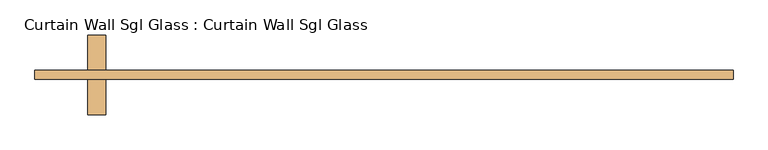
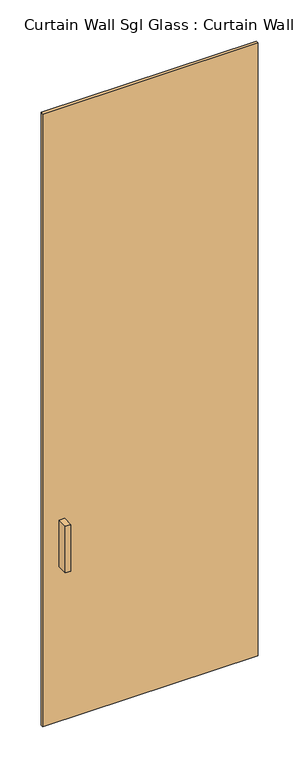
"""IFC4 building model written with IfcOpenShell, lengths in millimetres: door geometry, Curtain Wall Sgl Glass : Curtain Wall Sgl Glass."""

import ifcopenshell
import ifcopenshell.guid

model = None  # the IFC model being written
_history = None  # IfcOwnerHistory: only IFC2X3 demands one
_inside = {}  # id of a spatial element -> (the spatial element, [elements in it])
_under = {}  # id of a project, library or spatial element -> (it, [spatial elements below it])
_declared = {}  # id of a project -> (the project, [libraries it declares])
_typed = {}  # id of a type object -> (the type object, [elements of that type])
_made_of = {}  # id of a material, layer set ... -> (it, [elements and type objects made of it])


def new_model(schema):
    """Start an empty IFC model of exactly this schema.

    Asked for "IFC4X3", IfcOpenShell would pick the latest addendum, in which some entities
    have other attributes; the version numbers below select the first issue.
    IFC2X3 requires an IfcOwnerHistory on every rooted entity: one is made here for all.
    """
    global model, _history
    if schema == "IFC4X3":
        model = ifcopenshell.file(schema_version=(4, 3, 0, 0))
    else:
        model = ifcopenshell.file(schema=schema)
    _inside.clear()
    _under.clear()
    _declared.clear()
    _typed.clear()
    _made_of.clear()
    _history = None
    if model.schema == "IFC2X3":
        org = make("IfcOrganization", Name="unknown")
        user = make(
            "IfcPersonAndOrganization",
            ThePerson=make("IfcPerson", FamilyName="unknown"),
            TheOrganization=org,
        )
        app = make(
            "IfcApplication",
            ApplicationDeveloper=org,
            Version="unknown",
            ApplicationFullName="unknown",
            ApplicationIdentifier="unknown",
        )
        _history = make(
            "IfcOwnerHistory",
            OwningUser=user,
            OwningApplication=app,
            ChangeAction="ADDED",
            CreationDate=0,
        )
    return model


def make(cls, **values):
    """One entity of the class cls with the attributes given. An attribute that is None is left unset."""
    return model.create_entity(
        cls, **{name: value for name, value in values.items() if value is not None}
    )


def rooted(cls, **values):
    """An entity with a GlobalId (a new one), such as an element, a storey or a relation."""
    return make(cls, GlobalId=ifcopenshell.guid.new(), OwnerHistory=_history, **values)


def si_unit(unit_type, name, prefix=None):
    """IfcSIUnit, for example si_unit("LENGTHUNIT", "METRE", prefix="MILLI")."""
    return make("IfcSIUnit", UnitType=unit_type, Prefix=prefix, Name=name)


def assignment(units):
    """IfcUnitAssignment: the units of a project."""
    return None if units is None else make("IfcUnitAssignment", Units=units)


def point(xyz):
    """IfcCartesianPoint."""
    return None if xyz is None else make("IfcCartesianPoint", Coordinates=xyz)


def direction(xyz):
    """IfcDirection."""
    return None if xyz is None else make("IfcDirection", DirectionRatios=xyz)


def frame(location, z_axis=None, x_axis=None):
    """IfcAxis2Placement3D, a coordinate frame: its origin and axes. An axis left out is left unset."""
    return make(
        "IfcAxis2Placement3D",
        Location=point(location),
        Axis=direction(z_axis),
        RefDirection=direction(x_axis),
    )


def origin():
    """The frame at (0, 0, 0) with its axes left unset."""
    return frame((0.0, 0.0, 0.0))


def origin_with_axes():
    """The frame at (0, 0, 0) with the z axis (0, 0, 1) and the x axis (1, 0, 0) written out."""
    return frame((0.0, 0.0, 0.0), z_axis=(0.0, 0.0, 1.0), x_axis=(1.0, 0.0, 0.0))


def place(relative_to, where):
    """IfcLocalPlacement: puts the frame where relative to a parent placement (None: the world)."""
    return make(
        "IfcLocalPlacement", PlacementRelTo=relative_to, RelativePlacement=where
    )


def context(
    kind, dimensions, precision=None, world=None, true_north=None, identifier=None
):
    """IfcGeometricRepresentationContext, for example the 3D "Model" context."""
    return make(
        "IfcGeometricRepresentationContext",
        ContextIdentifier=identifier,
        ContextType=kind,
        CoordinateSpaceDimension=dimensions,
        Precision=precision,
        WorldCoordinateSystem=world,
        TrueNorth=true_north,
    )


def project(units=None, contexts=None):
    """IfcProject with its units and contexts."""
    return rooted(
        "IfcProject",
        Name="project",
        RepresentationContexts=contexts,
        UnitsInContext=assignment(units),
    )


def spatial(cls, under=None, at=None, **own):
    """A site, building, storey or space (cls), placed at a placement, below another one or the project."""
    s = rooted(cls, ObjectPlacement=at, **own)
    if under is not None:
        _under.setdefault(under.id(), (under, []))[1].append(s)
    return s


def polyline(points):
    """IfcPolyline through the points."""
    return make("IfcPolyline", Points=[point(p) for p in points])


def outline(outer, holes=None, kind="AREA"):
    """IfcArbitraryClosedProfileDef: a profile drawn as a closed curve; with holes, ...WithVoids."""
    if holes is None:
        return make("IfcArbitraryClosedProfileDef", ProfileType=kind, OuterCurve=outer)
    return make(
        "IfcArbitraryProfileDefWithVoids",
        ProfileType=kind,
        OuterCurve=outer,
        InnerCurves=holes,
    )


def extrude(swept, where, along, depth):
    """IfcExtrudedAreaSolid: the profile swept, set in the frame where, extruded along a direction by depth."""
    return make(
        "IfcExtrudedAreaSolid",
        SweptArea=swept,
        Position=where,
        ExtrudedDirection=direction(along),
        Depth=depth,
    )


def shape(context_of_items, identifier, shape_type, items):
    """IfcShapeRepresentation: the items that make up one representation, for example the "Body"."""
    return make(
        "IfcShapeRepresentation",
        ContextOfItems=context_of_items,
        RepresentationIdentifier=identifier,
        RepresentationType=shape_type,
        Items=items,
    )


def source(mapping_origin, context_of_items, identifier, shape_type, items):
    """IfcRepresentationMap: a shape defined once, which mapped items show again and again."""
    return make(
        "IfcRepresentationMap",
        MappingOrigin=mapping_origin,
        MappedRepresentation=shape(context_of_items, identifier, shape_type, items),
    )


def transform(
    local_origin,
    x_axis=None,
    y_axis=None,
    z_axis=None,
    scale=None,
    scale2=None,
    scale3=None,
    uniform=True,
):
    """IfcCartesianTransformationOperator3D, or its non-uniform kind. x_axis, y_axis, z_axis: its Axis1, 2, 3."""
    if uniform:
        return make(
            "IfcCartesianTransformationOperator3D",
            Axis1=direction(x_axis),
            Axis2=direction(y_axis),
            LocalOrigin=point(local_origin),
            Scale=scale,
            Axis3=direction(z_axis),
        )
    return make(
        "IfcCartesianTransformationOperator3DnonUniform",
        Axis1=direction(x_axis),
        Axis2=direction(y_axis),
        LocalOrigin=point(local_origin),
        Scale=scale,
        Axis3=direction(z_axis),
        Scale2=scale2,
        Scale3=scale3,
    )


def mapped(mapping_source, mapping_target):
    """IfcMappedItem: shows the shape of a source again, moved by a transform."""
    return make(
        "IfcMappedItem", MappingSource=mapping_source, MappingTarget=mapping_target
    )


def made_of(thing, what):
    """Note that an element or type object is made of a material, layer set ...; save() writes the relation."""
    if what is not None:
        _made_of.setdefault(what.id(), (what, []))[1].append(thing)
    return thing


def element(
    cls,
    number,
    at=None,
    inside=None,
    cuts=None,
    type_object=None,
    material=None,
    context=None,
    identifier="Body",
    shape_type=None,
    held_by="IfcProductDefinitionShape",
    body=None,
    shapes=None,
    **own,
):
    """One element of the class cls, such as IfcWall. Its Tag is "e" and its number.

    at: its placement. inside: the storey or other place that contains it. cuts: it is an
    opening in that element (IfcRelVoidsElement). A single representation is given by context,
    identifier, shape_type and body (its items); several are given by shapes. held_by: the class
    of the entity that holds the representations. save() writes the other relations.
    """
    e = rooted(cls, Tag="e%d" % number, ObjectPlacement=at, **own)
    if body is not None:
        shapes = [shape(context, identifier, shape_type, body)]
    if shapes is not None:
        e.Representation = make(held_by, Representations=shapes)
    if inside is not None:
        _inside.setdefault(inside.id(), (inside, []))[1].append(e)
    if cuts is not None:
        rooted(
            "IfcRelVoidsElement", RelatingBuildingElement=cuts, RelatedOpeningElement=e
        )
    if type_object is not None:
        _typed.setdefault(type_object.id(), (type_object, []))[1].append(e)
    return made_of(e, material)


def aggregate(whole, parts):
    """IfcRelAggregates: a whole, such as a stair, and the parts it consists of."""
    return rooted("IfcRelAggregates", RelatingObject=whole, RelatedObjects=parts)


def save(model, path):
    """Write the relations noted so far, then the file.

    IfcRelAggregates (storeys below a building ...), IfcRelContainedInSpatialStructure (elements
    in a storey), IfcRelDefinesByType, IfcRelAssociatesMaterial and IfcRelDeclares: one each for
    every whole, place, type object, material and project.
    """
    for whole, parts in _under.values():
        aggregate(whole, parts)
    for where, things in _inside.values():
        rooted(
            "IfcRelContainedInSpatialStructure",
            RelatedElements=things,
            RelatingStructure=where,
        )
    for kind, things in _typed.values():
        rooted("IfcRelDefinesByType", RelatedObjects=things, RelatingType=kind)
    for what, things in _made_of.values():
        rooted("IfcRelAssociatesMaterial", RelatedObjects=things, RelatingMaterial=what)
    for by, libraries in _declared.values():
        rooted("IfcRelDeclares", RelatingContext=by, RelatedDefinitions=libraries)
    model.write(path)


def curtain_wall_sgl_glass_curtain_wall_sgl_glass_6f19eea7(model_context):
    return source(origin(), model_context, "Body", "SweptSolid", [
        extrude(outline(polyline([(-399.5964286, -12.7), (-424.9964286, -12.7), (-424.9964286, 38.1), (-399.5964286, 38.1), (-399.5964286, -12.7)])), frame((0.0, 0.0, 762.0), z_axis=(0.0, 0.0, 1.0), x_axis=(1.0, 0.0, 0.0)), (0.0, 0.0, 1.0), 228.6),
        extrude(outline(polyline([(-424.9964286, 101.6), (-399.5964286, 101.6), (-399.5964286, 50.8), (-424.9964286, 50.8), (-424.9964286, 101.6)])), frame((0.0, 0.0, 762.0), z_axis=(0.0, 0.0, 1.0), x_axis=(1.0, 0.0, 0.0)), (0.0, 0.0, 1.0), 228.6),
        extrude(outline(polyline([(501.1964286, 50.8), (501.1964286, 38.1), (-501.1964286, 38.1), (-501.1964286, 50.8), (501.1964286, 50.8)])), origin_with_axes(), (0.0, 0.0, 1.0), 3016.25),
    ])


if __name__ == "__main__":
    model = new_model("IFC4")
    model_context = context("Model", 3, world=origin())
    ifc_project = project(units=[si_unit("LENGTHUNIT", "METRE", prefix="MILLI")], contexts=[model_context])
    site = spatial("IfcSite", under=ifc_project)
    building = spatial("IfcBuilding", under=site)
    placement = place(None, origin())
    curtain_wall_sgl_glass_curtain_wall_sgl_glass_shape = curtain_wall_sgl_glass_curtain_wall_sgl_glass_6f19eea7(model_context)
    element("IfcDoor", 1, ObjectType="Curtain Wall Sgl Glass : Curtain Wall Sgl Glass", at=placement, inside=building, context=model_context, shape_type="MappedRepresentation", body=[
        mapped(curtain_wall_sgl_glass_curtain_wall_sgl_glass_shape, transform((0.0, 0.0, 0.0), x_axis=(1.0, 0.0, 0.0), y_axis=(0.0, 1.0, 0.0), z_axis=(0.0, 0.0, 1.0))),
    ])
    save(model, "model.ifc")

# Revit data of these elements
# Type "Curtain Wall Sgl Glass : Curtain Wall Sgl Glass"
#   Type Mark = "8"
#   Assembly Code = "B2030100"
#   Offset = 50.80 mm
#   Function = 1
#   Handle Material = Metal - Aluminum
#   Glazing Material = Glass
# Element 1 (IfcDoor, "Curtain Wall Sgl Glass : Curtain Wall Sgl Glass")
#   Materials on its faces: "Metal - Aluminum", "Glass"
# Materials
#   "Metal - Aluminum": class "Metal", colour RGB 247 247 247, transparency 0
#   "Glass": class "Unassigned", colour RGB 0 0 255, transparency 0.75
